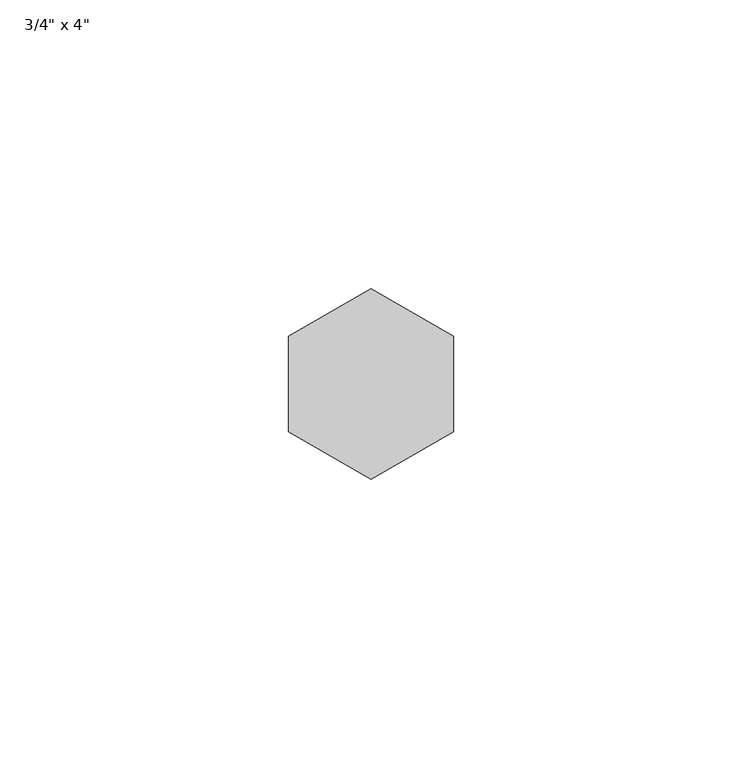
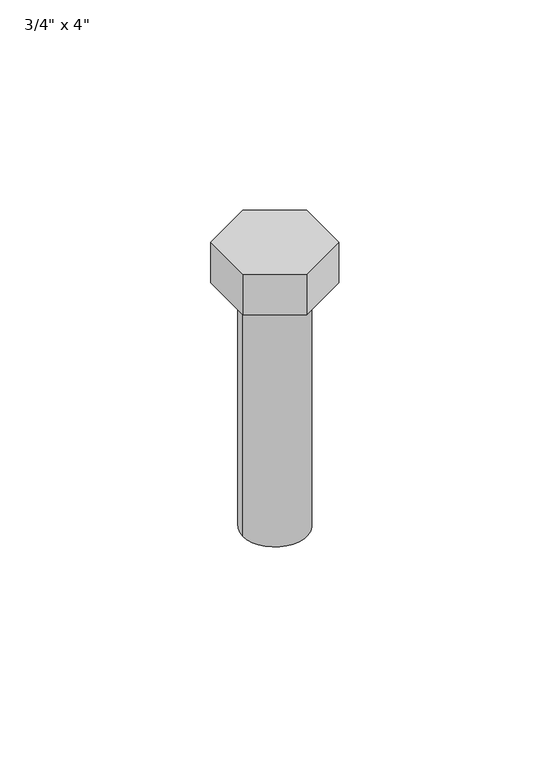
"""IFC4 building model written with IfcOpenShell, lengths in millimetres: proxy geometry."""

import ifcopenshell
import ifcopenshell.guid

model = None  # the IFC model being written
_history = None  # IfcOwnerHistory: only IFC2X3 demands one
_inside = {}  # id of a spatial element -> (the spatial element, [elements in it])
_under = {}  # id of a project, library or spatial element -> (it, [spatial elements below it])
_declared = {}  # id of a project -> (the project, [libraries it declares])
_typed = {}  # id of a type object -> (the type object, [elements of that type])
_made_of = {}  # id of a material, layer set ... -> (it, [elements and type objects made of it])


def new_model(schema):
    """Start an empty IFC model of exactly this schema.

    Asked for "IFC4X3", IfcOpenShell would pick the latest addendum, in which some entities
    have other attributes; the version numbers below select the first issue.
    IFC2X3 requires an IfcOwnerHistory on every rooted entity: one is made here for all.
    """
    global model, _history
    if schema == "IFC4X3":
        model = ifcopenshell.file(schema_version=(4, 3, 0, 0))
    else:
        model = ifcopenshell.file(schema=schema)
    _inside.clear()
    _under.clear()
    _declared.clear()
    _typed.clear()
    _made_of.clear()
    _history = None
    if model.schema == "IFC2X3":
        org = make("IfcOrganization", Name="unknown")
        user = make(
            "IfcPersonAndOrganization",
            ThePerson=make("IfcPerson", FamilyName="unknown"),
            TheOrganization=org,
        )
        app = make(
            "IfcApplication",
            ApplicationDeveloper=org,
            Version="unknown",
            ApplicationFullName="unknown",
            ApplicationIdentifier="unknown",
        )
        _history = make(
            "IfcOwnerHistory",
            OwningUser=user,
            OwningApplication=app,
            ChangeAction="ADDED",
            CreationDate=0,
        )
    return model


def make(cls, **values):
    """One entity of the class cls with the attributes given. An attribute that is None is left unset."""
    return model.create_entity(
        cls, **{name: value for name, value in values.items() if value is not None}
    )


def rooted(cls, **values):
    """An entity with a GlobalId (a new one), such as an element, a storey or a relation."""
    return make(cls, GlobalId=ifcopenshell.guid.new(), OwnerHistory=_history, **values)


def si_unit(unit_type, name, prefix=None):
    """IfcSIUnit, for example si_unit("LENGTHUNIT", "METRE", prefix="MILLI")."""
    return make("IfcSIUnit", UnitType=unit_type, Prefix=prefix, Name=name)


def assignment(units):
    """IfcUnitAssignment: the units of a project."""
    return None if units is None else make("IfcUnitAssignment", Units=units)


def point(xyz):
    """IfcCartesianPoint."""
    return None if xyz is None else make("IfcCartesianPoint", Coordinates=xyz)


def direction(xyz):
    """IfcDirection."""
    return None if xyz is None else make("IfcDirection", DirectionRatios=xyz)


def frame(location, z_axis=None, x_axis=None):
    """IfcAxis2Placement3D, a coordinate frame: its origin and axes. An axis left out is left unset."""
    return make(
        "IfcAxis2Placement3D",
        Location=point(location),
        Axis=direction(z_axis),
        RefDirection=direction(x_axis),
    )


def frame_2d(location, x_axis=None):
    """IfcAxis2Placement2D, a coordinate frame in the plane: its origin and x axis."""
    return make(
        "IfcAxis2Placement2D", Location=point(location), RefDirection=direction(x_axis)
    )


def origin():
    """The frame at (0, 0, 0) with its axes left unset."""
    return frame((0.0, 0.0, 0.0))


def origin_with_axes():
    """The frame at (0, 0, 0) with the z axis (0, 0, 1) and the x axis (1, 0, 0) written out."""
    return frame((0.0, 0.0, 0.0), z_axis=(0.0, 0.0, 1.0), x_axis=(1.0, 0.0, 0.0))


def origin_2d():
    """The frame at (0, 0) in the plane with its x axis left unset."""
    return frame_2d((0.0, 0.0))


def place(relative_to, where):
    """IfcLocalPlacement: puts the frame where relative to a parent placement (None: the world)."""
    return make(
        "IfcLocalPlacement", PlacementRelTo=relative_to, RelativePlacement=where
    )


def context(
    kind, dimensions, precision=None, world=None, true_north=None, identifier=None
):
    """IfcGeometricRepresentationContext, for example the 3D "Model" context."""
    return make(
        "IfcGeometricRepresentationContext",
        ContextIdentifier=identifier,
        ContextType=kind,
        CoordinateSpaceDimension=dimensions,
        Precision=precision,
        WorldCoordinateSystem=world,
        TrueNorth=true_north,
    )


def project(units=None, contexts=None):
    """IfcProject with its units and contexts."""
    return rooted(
        "IfcProject",
        Name="project",
        RepresentationContexts=contexts,
        UnitsInContext=assignment(units),
    )


def spatial(cls, under=None, at=None, **own):
    """A site, building, storey or space (cls), placed at a placement, below another one or the project."""
    s = rooted(cls, ObjectPlacement=at, **own)
    if under is not None:
        _under.setdefault(under.id(), (under, []))[1].append(s)
    return s


def polyline(points):
    """IfcPolyline through the points."""
    return make("IfcPolyline", Points=[point(p) for p in points])


def circle_curve(where, radius):
    """IfcCircle in the frame where."""
    return make("IfcCircle", Position=where, Radius=radius)


def trimmed(basis, trim1, trim2, sense, master):
    """IfcTrimmedCurve: the piece of a basis curve between two trims."""
    return make(
        "IfcTrimmedCurve",
        BasisCurve=basis,
        Trim1=trim1,
        Trim2=trim2,
        SenseAgreement=sense,
        MasterRepresentation=master,
    )


def segment(curve, same_sense, transition):
    """IfcCompositeCurveSegment."""
    return make(
        "IfcCompositeCurveSegment",
        Transition=transition,
        SameSense=same_sense,
        ParentCurve=curve,
    )


def composite_curve(segments, self_intersect=None):
    """IfcCompositeCurve: segments joined end to end."""
    return make("IfcCompositeCurve", Segments=segments, SelfIntersect=self_intersect)


def outline(outer, holes=None, kind="AREA"):
    """IfcArbitraryClosedProfileDef: a profile drawn as a closed curve; with holes, ...WithVoids."""
    if holes is None:
        return make("IfcArbitraryClosedProfileDef", ProfileType=kind, OuterCurve=outer)
    return make(
        "IfcArbitraryProfileDefWithVoids",
        ProfileType=kind,
        OuterCurve=outer,
        InnerCurves=holes,
    )


def extrude(swept, where, along, depth):
    """IfcExtrudedAreaSolid: the profile swept, set in the frame where, extruded along a direction by depth."""
    return make(
        "IfcExtrudedAreaSolid",
        SweptArea=swept,
        Position=where,
        ExtrudedDirection=direction(along),
        Depth=depth,
    )


def shape(context_of_items, identifier, shape_type, items):
    """IfcShapeRepresentation: the items that make up one representation, for example the "Body"."""
    return make(
        "IfcShapeRepresentation",
        ContextOfItems=context_of_items,
        RepresentationIdentifier=identifier,
        RepresentationType=shape_type,
        Items=items,
    )


def source(mapping_origin, context_of_items, identifier, shape_type, items):
    """IfcRepresentationMap: a shape defined once, which mapped items show again and again."""
    return make(
        "IfcRepresentationMap",
        MappingOrigin=mapping_origin,
        MappedRepresentation=shape(context_of_items, identifier, shape_type, items),
    )


def transform(
    local_origin,
    x_axis=None,
    y_axis=None,
    z_axis=None,
    scale=None,
    scale2=None,
    scale3=None,
    uniform=True,
):
    """IfcCartesianTransformationOperator3D, or its non-uniform kind. x_axis, y_axis, z_axis: its Axis1, 2, 3."""
    if uniform:
        return make(
            "IfcCartesianTransformationOperator3D",
            Axis1=direction(x_axis),
            Axis2=direction(y_axis),
            LocalOrigin=point(local_origin),
            Scale=scale,
            Axis3=direction(z_axis),
        )
    return make(
        "IfcCartesianTransformationOperator3DnonUniform",
        Axis1=direction(x_axis),
        Axis2=direction(y_axis),
        LocalOrigin=point(local_origin),
        Scale=scale,
        Axis3=direction(z_axis),
        Scale2=scale2,
        Scale3=scale3,
    )


def mapped(mapping_source, mapping_target):
    """IfcMappedItem: shows the shape of a source again, moved by a transform."""
    return make(
        "IfcMappedItem", MappingSource=mapping_source, MappingTarget=mapping_target
    )


def made_of(thing, what):
    """Note that an element or type object is made of a material, layer set ...; save() writes the relation."""
    if what is not None:
        _made_of.setdefault(what.id(), (what, []))[1].append(thing)
    return thing


def element(
    cls,
    number,
    at=None,
    inside=None,
    cuts=None,
    type_object=None,
    material=None,
    context=None,
    identifier="Body",
    shape_type=None,
    held_by="IfcProductDefinitionShape",
    body=None,
    shapes=None,
    **own,
):
    """One element of the class cls, such as IfcWall. Its Tag is "e" and its number.

    at: its placement. inside: the storey or other place that contains it. cuts: it is an
    opening in that element (IfcRelVoidsElement). A single representation is given by context,
    identifier, shape_type and body (its items); several are given by shapes. held_by: the class
    of the entity that holds the representations. save() writes the other relations.
    """
    e = rooted(cls, Tag="e%d" % number, ObjectPlacement=at, **own)
    if body is not None:
        shapes = [shape(context, identifier, shape_type, body)]
    if shapes is not None:
        e.Representation = make(held_by, Representations=shapes)
    if inside is not None:
        _inside.setdefault(inside.id(), (inside, []))[1].append(e)
    if cuts is not None:
        rooted(
            "IfcRelVoidsElement", RelatingBuildingElement=cuts, RelatedOpeningElement=e
        )
    if type_object is not None:
        _typed.setdefault(type_object.id(), (type_object, []))[1].append(e)
    return made_of(e, material)


def aggregate(whole, parts):
    """IfcRelAggregates: a whole, such as a stair, and the parts it consists of."""
    return rooted("IfcRelAggregates", RelatingObject=whole, RelatedObjects=parts)


def save(model, path):
    """Write the relations noted so far, then the file.

    IfcRelAggregates (storeys below a building ...), IfcRelContainedInSpatialStructure (elements
    in a storey), IfcRelDefinesByType, IfcRelAssociatesMaterial and IfcRelDeclares: one each for
    every whole, place, type object, material and project.
    """
    for whole, parts in _under.values():
        aggregate(whole, parts)
    for where, things in _inside.values():
        rooted(
            "IfcRelContainedInSpatialStructure",
            RelatedElements=things,
            RelatingStructure=where,
        )
    for kind, things in _typed.values():
        rooted("IfcRelDefinesByType", RelatedObjects=things, RelatingType=kind)
    for what, things in _made_of.values():
        rooted("IfcRelAssociatesMaterial", RelatedObjects=things, RelatingMaterial=what)
    for by, libraries in _declared.values():
        rooted("IfcRelDeclares", RelatingContext=by, RelatedDefinitions=libraries)
    model.write(path)


def proxy_883de4b5(model_context):
    return source(origin(), model_context, "Body", "SweptSolid", [
        extrude(outline(polyline([(-14.2875, 8.248892), (0.0, 16.4977839), (14.2875, 8.248892), (14.2875, -8.248892), (0.0, -16.4977839), (-14.2875, -8.248892), (-14.2875, 8.248892)])), origin_with_axes(), (0.0, 0.0, 1.0), 12.7),
        extrude(outline(composite_curve([segment(trimmed(circle_curve(origin_2d(), 9.525), [point((-9.525, 0.0))], [point((9.525, 0.0))], False, "CARTESIAN"), True, "CONTINUOUS"), segment(trimmed(circle_curve(origin_2d(), 9.525), [point((9.525, 0.0))], [point((-9.525, 0.0))], False, "CARTESIAN"), True, "CONTINUOUS")], self_intersect=False)), frame((0.0, 0.0, -76.2), z_axis=(0.0, 0.0, 1.0), x_axis=(1.0, 0.0, 0.0)), (0.0, 0.0, 1.0), 76.2),
    ])


if __name__ == "__main__":
    model = new_model("IFC4")
    model_context = context("Model", 3, world=origin())
    ifc_project = project(units=[si_unit("LENGTHUNIT", "METRE", prefix="MILLI")], contexts=[model_context])
    site = spatial("IfcSite", under=ifc_project)
    building = spatial("IfcBuilding", under=site)
    placement = place(None, origin())
    proxy_shape = proxy_883de4b5(model_context)
    element("IfcBuildingElementProxy", 1, Name="050523 - W_P_C - Fastenings - Lag Bolt or Thru Bolt : 3/4\" x 4\"", ObjectType="050523 - W_P_C - Fastenings - Lag Bolt or Thru Bolt : 3/4\" x 4\"", at=placement, inside=building, context=model_context, shape_type="MappedRepresentation", body=[
        mapped(proxy_shape, transform((0.0, 0.0, 0.0), x_axis=(1.0, 0.0, 0.0), y_axis=(0.0, 1.0, 0.0), z_axis=(0.0, 0.0, 1.0))),
    ])
    save(model, "model.ifc")

# Revit data of these elements
# Type "050523 - W_P_C - Fastenings - Lag Bolt or Thru Bolt : 3/4\" x 4\""
#   Thickness_of_Substrate [instance default] = 0' - 1"
#   Side = 0' - 0.65039"
#   Radius = 0' - 0 3/8"
#   Length = 0' - 3"
#   Head Size = 0' - 1 1/8"
#   Head Radius = 0' - 0 9/16"
#   Head Height = 0' - 0 1/2"
#   Diameter = 0' - 0 3/4"
#   Default Elevation = 4' - 0"
#   Nut_Visibility [instance default] = yes
#   Bolt Material (Size) = EXPOSED LAG BOLTS - SEE STRUCT.
# Element 1 (IfcBuildingElementProxy, "050523 - W_P_C - Fastenings - Lag Bolt or Thru Bolt : 3/4\" x 4\"")
#   Nut_Visibility = no
#   Materials on its faces: "EXPOSED LAG BOLTS - SEE STRUCT."
# Materials
#   "EXPOSED LAG BOLTS - SEE STRUCT.": class "Generic", colour RGB 120 120 120, transparency 0, Cost = 0
